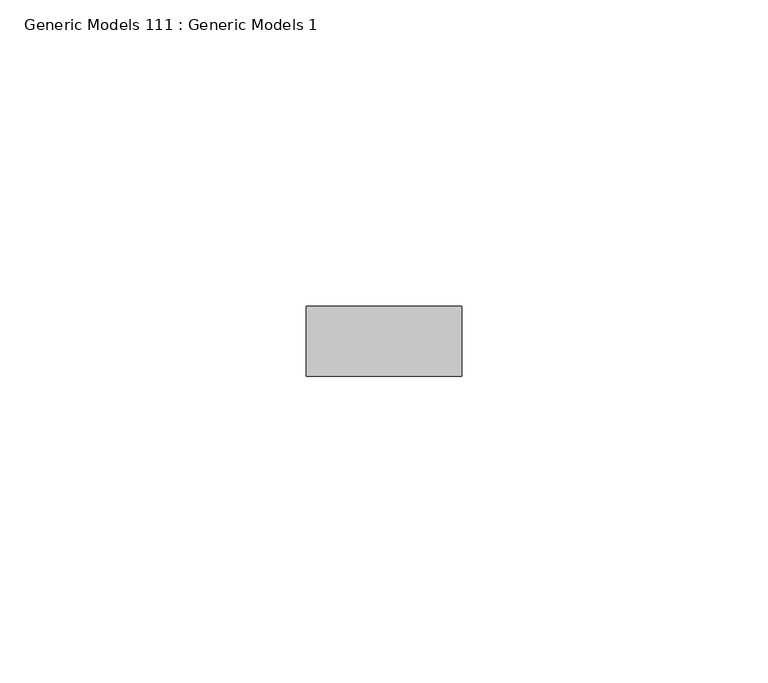
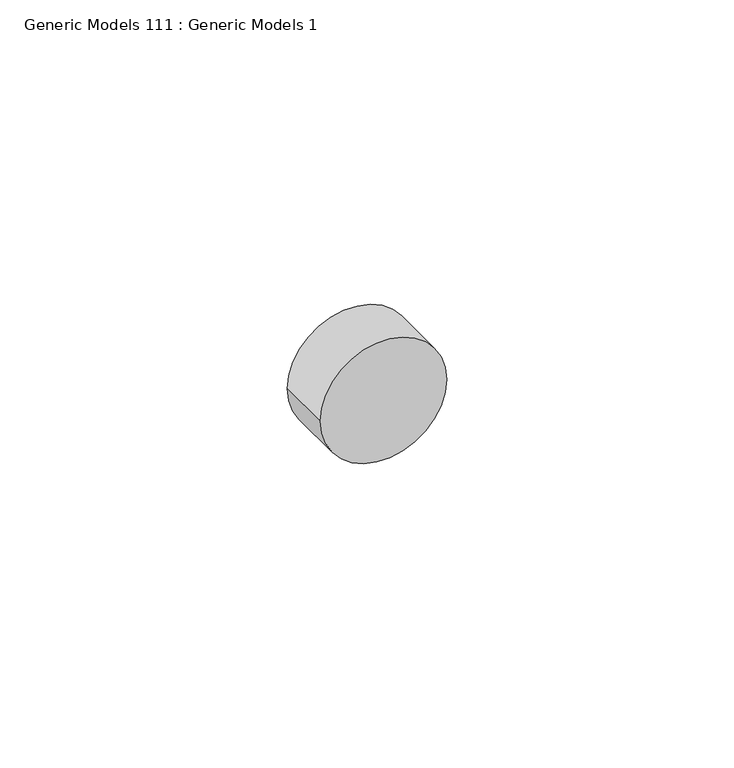
"""IFC4 building model written with IfcOpenShell, lengths in millimetres: proxy geometry, Generic Models 111 : Generic Models 1."""

from ifc_helpers import new_model, si_unit, point, frame, frame_2d, origin, place, context, project, spatial, circle_curve, trimmed, segment, composite_curve, outline, extrude, source, transform, mapped, element, save


def generic_models_111_generic_models_1_badaa977(model_context):
    return source(origin(), model_context, "Body", "SweptSolid", [
        extrude(outline(composite_curve([segment(trimmed(circle_curve(frame_2d((37688.9033735, 6459.3346014)), 12.7), [point((37688.9033735, 6472.0346014))], [point((37688.9033735, 6446.6346014))], False, "CARTESIAN"), True, "CONTINUOUS"), segment(trimmed(circle_curve(frame_2d((37688.9033735, 6459.3346014)), 12.7), [point((37688.9033735, 6446.6346014))], [point((37688.9033735, 6472.0346014))], False, "CARTESIAN"), True, "CONTINUOUS")], self_intersect=False)), frame((0.0, 1836.9202358, 0.0), z_axis=(0.0, 1.0, 0.0), x_axis=(0.0, 0.0, 1.0)), (0.0, 0.0, 1.0), 11.4464372),
    ])


if __name__ == "__main__":
    model = new_model("IFC4")
    model_context = context("Model", 3, world=origin())
    ifc_project = project(units=[si_unit("LENGTHUNIT", "METRE", prefix="MILLI")], contexts=[model_context])
    site = spatial("IfcSite", under=ifc_project)
    building = spatial("IfcBuilding", under=site)
    placement = place(None, origin())
    generic_models_111_generic_models_1_shape = generic_models_111_generic_models_1_badaa977(model_context)
    element("IfcBuildingElementProxy", 1, Name="Generic Models 111 : Generic Models 1", ObjectType="Generic Models 111 : Generic Models 1", at=placement, inside=building, context=model_context, shape_type="MappedRepresentation", body=[
        mapped(generic_models_111_generic_models_1_shape, transform((0.0, 0.0, 0.0), x_axis=(1.0, 0.0, 0.0), y_axis=(0.0, 1.0, 0.0), z_axis=(0.0, 0.0, 1.0))),
    ])
    save(model, "model.ifc")

# Revit data of these elements
# Element 1 (IfcBuildingElementProxy, "Generic Models 111 : Generic Models 1")
#   Materials on its faces: "S.S. LAG BOLT - SEE STRUCT. DWGS"
# Materials
#   "S.S. LAG BOLT - SEE STRUCT. DWGS": class "Generic", colour RGB 120 120 120, transparency 0, Cost = 0
